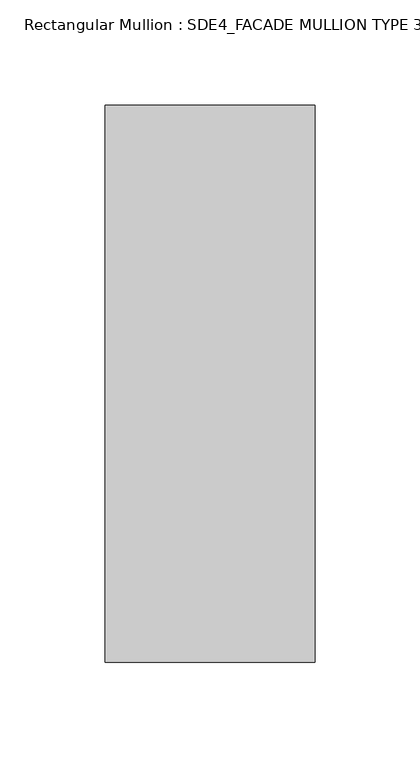
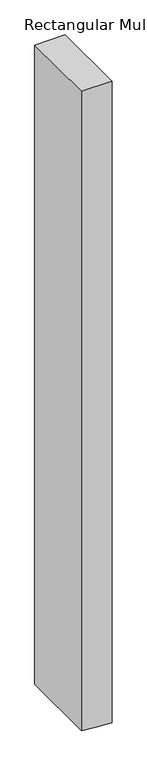
"""IFC4 building model written with IfcOpenShell, lengths in millimetres: member geometry, Rectangular Mullion : SDE4_FACADE MULLION TYPE 3."""

import ifcopenshell
import ifcopenshell.guid

model = None  # the IFC model being written
_history = None  # IfcOwnerHistory: only IFC2X3 demands one
_inside = {}  # id of a spatial element -> (the spatial element, [elements in it])
_under = {}  # id of a project, library or spatial element -> (it, [spatial elements below it])
_declared = {}  # id of a project -> (the project, [libraries it declares])
_typed = {}  # id of a type object -> (the type object, [elements of that type])
_made_of = {}  # id of a material, layer set ... -> (it, [elements and type objects made of it])


def new_model(schema):
    """Start an empty IFC model of exactly this schema.

    Asked for "IFC4X3", IfcOpenShell would pick the latest addendum, in which some entities
    have other attributes; the version numbers below select the first issue.
    IFC2X3 requires an IfcOwnerHistory on every rooted entity: one is made here for all.
    """
    global model, _history
    if schema == "IFC4X3":
        model = ifcopenshell.file(schema_version=(4, 3, 0, 0))
    else:
        model = ifcopenshell.file(schema=schema)
    _inside.clear()
    _under.clear()
    _declared.clear()
    _typed.clear()
    _made_of.clear()
    _history = None
    if model.schema == "IFC2X3":
        org = make("IfcOrganization", Name="unknown")
        user = make(
            "IfcPersonAndOrganization",
            ThePerson=make("IfcPerson", FamilyName="unknown"),
            TheOrganization=org,
        )
        app = make(
            "IfcApplication",
            ApplicationDeveloper=org,
            Version="unknown",
            ApplicationFullName="unknown",
            ApplicationIdentifier="unknown",
        )
        _history = make(
            "IfcOwnerHistory",
            OwningUser=user,
            OwningApplication=app,
            ChangeAction="ADDED",
            CreationDate=0,
        )
    return model


def make(cls, **values):
    """One entity of the class cls with the attributes given. An attribute that is None is left unset."""
    return model.create_entity(
        cls, **{name: value for name, value in values.items() if value is not None}
    )


def rooted(cls, **values):
    """An entity with a GlobalId (a new one), such as an element, a storey or a relation."""
    return make(cls, GlobalId=ifcopenshell.guid.new(), OwnerHistory=_history, **values)


def si_unit(unit_type, name, prefix=None):
    """IfcSIUnit, for example si_unit("LENGTHUNIT", "METRE", prefix="MILLI")."""
    return make("IfcSIUnit", UnitType=unit_type, Prefix=prefix, Name=name)


def assignment(units):
    """IfcUnitAssignment: the units of a project."""
    return None if units is None else make("IfcUnitAssignment", Units=units)


def point(xyz):
    """IfcCartesianPoint."""
    return None if xyz is None else make("IfcCartesianPoint", Coordinates=xyz)


def direction(xyz):
    """IfcDirection."""
    return None if xyz is None else make("IfcDirection", DirectionRatios=xyz)


def frame(location, z_axis=None, x_axis=None):
    """IfcAxis2Placement3D, a coordinate frame: its origin and axes. An axis left out is left unset."""
    return make(
        "IfcAxis2Placement3D",
        Location=point(location),
        Axis=direction(z_axis),
        RefDirection=direction(x_axis),
    )


def origin():
    """The frame at (0, 0, 0) with its axes left unset."""
    return frame((0.0, 0.0, 0.0))


def place(relative_to, where):
    """IfcLocalPlacement: puts the frame where relative to a parent placement (None: the world)."""
    return make(
        "IfcLocalPlacement", PlacementRelTo=relative_to, RelativePlacement=where
    )


def context(
    kind, dimensions, precision=None, world=None, true_north=None, identifier=None
):
    """IfcGeometricRepresentationContext, for example the 3D "Model" context."""
    return make(
        "IfcGeometricRepresentationContext",
        ContextIdentifier=identifier,
        ContextType=kind,
        CoordinateSpaceDimension=dimensions,
        Precision=precision,
        WorldCoordinateSystem=world,
        TrueNorth=true_north,
    )


def project(units=None, contexts=None):
    """IfcProject with its units and contexts."""
    return rooted(
        "IfcProject",
        Name="project",
        RepresentationContexts=contexts,
        UnitsInContext=assignment(units),
    )


def spatial(cls, under=None, at=None, **own):
    """A site, building, storey or space (cls), placed at a placement, below another one or the project."""
    s = rooted(cls, ObjectPlacement=at, **own)
    if under is not None:
        _under.setdefault(under.id(), (under, []))[1].append(s)
    return s


def polyline(points):
    """IfcPolyline through the points."""
    return make("IfcPolyline", Points=[point(p) for p in points])


def outline(outer, holes=None, kind="AREA"):
    """IfcArbitraryClosedProfileDef: a profile drawn as a closed curve; with holes, ...WithVoids."""
    if holes is None:
        return make("IfcArbitraryClosedProfileDef", ProfileType=kind, OuterCurve=outer)
    return make(
        "IfcArbitraryProfileDefWithVoids",
        ProfileType=kind,
        OuterCurve=outer,
        InnerCurves=holes,
    )


def extrude(swept, where, along, depth):
    """IfcExtrudedAreaSolid: the profile swept, set in the frame where, extruded along a direction by depth."""
    return make(
        "IfcExtrudedAreaSolid",
        SweptArea=swept,
        Position=where,
        ExtrudedDirection=direction(along),
        Depth=depth,
    )


def shape(context_of_items, identifier, shape_type, items):
    """IfcShapeRepresentation: the items that make up one representation, for example the "Body"."""
    return make(
        "IfcShapeRepresentation",
        ContextOfItems=context_of_items,
        RepresentationIdentifier=identifier,
        RepresentationType=shape_type,
        Items=items,
    )


def source(mapping_origin, context_of_items, identifier, shape_type, items):
    """IfcRepresentationMap: a shape defined once, which mapped items show again and again."""
    return make(
        "IfcRepresentationMap",
        MappingOrigin=mapping_origin,
        MappedRepresentation=shape(context_of_items, identifier, shape_type, items),
    )


def transform(
    local_origin,
    x_axis=None,
    y_axis=None,
    z_axis=None,
    scale=None,
    scale2=None,
    scale3=None,
    uniform=True,
):
    """IfcCartesianTransformationOperator3D, or its non-uniform kind. x_axis, y_axis, z_axis: its Axis1, 2, 3."""
    if uniform:
        return make(
            "IfcCartesianTransformationOperator3D",
            Axis1=direction(x_axis),
            Axis2=direction(y_axis),
            LocalOrigin=point(local_origin),
            Scale=scale,
            Axis3=direction(z_axis),
        )
    return make(
        "IfcCartesianTransformationOperator3DnonUniform",
        Axis1=direction(x_axis),
        Axis2=direction(y_axis),
        LocalOrigin=point(local_origin),
        Scale=scale,
        Axis3=direction(z_axis),
        Scale2=scale2,
        Scale3=scale3,
    )


def mapped(mapping_source, mapping_target):
    """IfcMappedItem: shows the shape of a source again, moved by a transform."""
    return make(
        "IfcMappedItem", MappingSource=mapping_source, MappingTarget=mapping_target
    )


def made_of(thing, what):
    """Note that an element or type object is made of a material, layer set ...; save() writes the relation."""
    if what is not None:
        _made_of.setdefault(what.id(), (what, []))[1].append(thing)
    return thing


def element(
    cls,
    number,
    at=None,
    inside=None,
    cuts=None,
    type_object=None,
    material=None,
    context=None,
    identifier="Body",
    shape_type=None,
    held_by="IfcProductDefinitionShape",
    body=None,
    shapes=None,
    **own,
):
    """One element of the class cls, such as IfcWall. Its Tag is "e" and its number.

    at: its placement. inside: the storey or other place that contains it. cuts: it is an
    opening in that element (IfcRelVoidsElement). A single representation is given by context,
    identifier, shape_type and body (its items); several are given by shapes. held_by: the class
    of the entity that holds the representations. save() writes the other relations.
    """
    e = rooted(cls, Tag="e%d" % number, ObjectPlacement=at, **own)
    if body is not None:
        shapes = [shape(context, identifier, shape_type, body)]
    if shapes is not None:
        e.Representation = make(held_by, Representations=shapes)
    if inside is not None:
        _inside.setdefault(inside.id(), (inside, []))[1].append(e)
    if cuts is not None:
        rooted(
            "IfcRelVoidsElement", RelatingBuildingElement=cuts, RelatedOpeningElement=e
        )
    if type_object is not None:
        _typed.setdefault(type_object.id(), (type_object, []))[1].append(e)
    return made_of(e, material)


def aggregate(whole, parts):
    """IfcRelAggregates: a whole, such as a stair, and the parts it consists of."""
    return rooted("IfcRelAggregates", RelatingObject=whole, RelatedObjects=parts)


def save(model, path):
    """Write the relations noted so far, then the file.

    IfcRelAggregates (storeys below a building ...), IfcRelContainedInSpatialStructure (elements
    in a storey), IfcRelDefinesByType, IfcRelAssociatesMaterial and IfcRelDeclares: one each for
    every whole, place, type object, material and project.
    """
    for whole, parts in _under.values():
        aggregate(whole, parts)
    for where, things in _inside.values():
        rooted(
            "IfcRelContainedInSpatialStructure",
            RelatedElements=things,
            RelatingStructure=where,
        )
    for kind, things in _typed.values():
        rooted("IfcRelDefinesByType", RelatedObjects=things, RelatingType=kind)
    for what, things in _made_of.values():
        rooted("IfcRelAssociatesMaterial", RelatedObjects=things, RelatingMaterial=what)
    for by, libraries in _declared.values():
        rooted("IfcRelDeclares", RelatingContext=by, RelatedDefinitions=libraries)
    model.write(path)


def rectangular_mullion_sde4_facade_mullion_type_3_06bc7ad0(model_context):
    return source(origin(), model_context, "Body", "SweptSolid", [
        extrude(outline(polyline([(0.0, 50.0), (0.0, -50.0), (-2211.4836429, -50.0), (-2215.5497219, 3.056508), (-2219.1473192, 50.0), (0.0, 50.0)])), frame((0.0, -132.5, 0.0), z_axis=(0.0, 1.0, 0.0), x_axis=(0.0, 0.0, 1.0)), (0.0, 0.0, 1.0), 265.0),
    ])


if __name__ == "__main__":
    model = new_model("IFC4")
    model_context = context("Model", 3, world=origin())
    ifc_project = project(units=[si_unit("LENGTHUNIT", "METRE", prefix="MILLI")], contexts=[model_context])
    site = spatial("IfcSite", under=ifc_project)
    building = spatial("IfcBuilding", under=site)
    placement = place(None, origin())
    rectangular_mullion_sde4_facade_mullion_type_3_shape = rectangular_mullion_sde4_facade_mullion_type_3_06bc7ad0(model_context)
    element("IfcMember", 1, ObjectType="Rectangular Mullion : SDE4_FACADE MULLION TYPE 3", at=placement, inside=building, context=model_context, shape_type="MappedRepresentation", body=[
        mapped(rectangular_mullion_sde4_facade_mullion_type_3_shape, transform((0.0, 0.0, 0.0), x_axis=(1.0, 0.0, 0.0), y_axis=(0.0, 1.0, 0.0), z_axis=(0.0, 0.0, 1.0))),
    ])
    save(model, "model.ifc")

# Revit data of these elements
# Type "Rectangular Mullion : SDE4_FACADE MULLION TYPE 3"
#   built-in parameter 1007322 = 0.869423 (stored number, unit not read)
#   built-in parameter 1007321 = 0.164042 (stored number, unit not read)
#   built-in parameter 1007320 = 0.164042 (stored number, unit not read)
